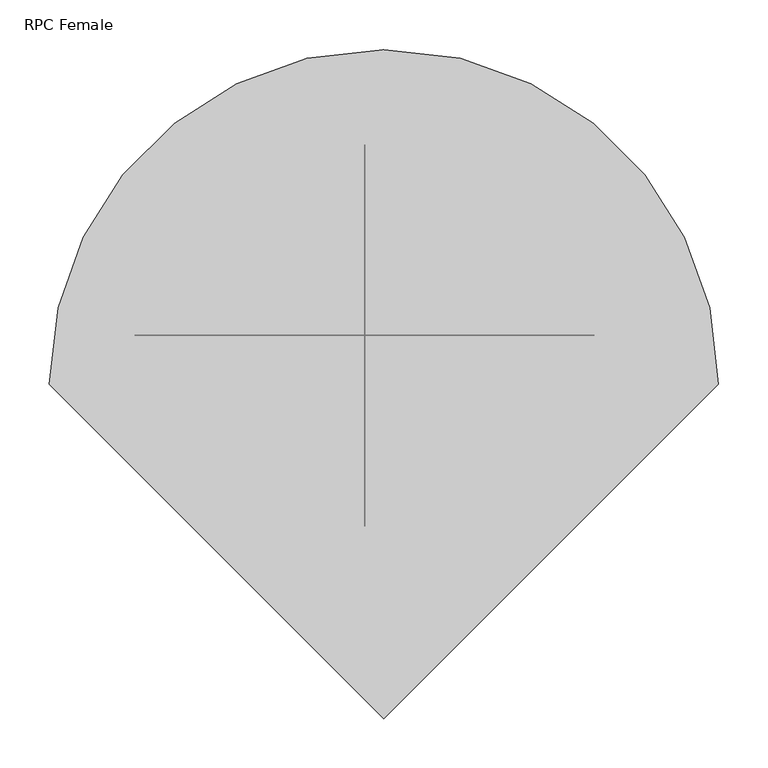
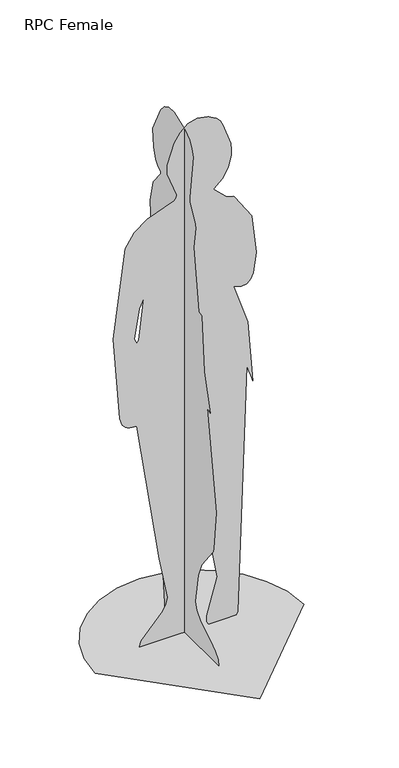
"""IFC4 building model written with IfcOpenShell, lengths in millimetres: proxy geometry, RPC Female : YinYin."""

import ifcopenshell
import ifcopenshell.guid

model = None  # the IFC model being written
_history = None  # IfcOwnerHistory: only IFC2X3 demands one
_inside = {}  # id of a spatial element -> (the spatial element, [elements in it])
_under = {}  # id of a project, library or spatial element -> (it, [spatial elements below it])
_declared = {}  # id of a project -> (the project, [libraries it declares])
_typed = {}  # id of a type object -> (the type object, [elements of that type])
_made_of = {}  # id of a material, layer set ... -> (it, [elements and type objects made of it])


def new_model(schema):
    """Start an empty IFC model of exactly this schema.

    Asked for "IFC4X3", IfcOpenShell would pick the latest addendum, in which some entities
    have other attributes; the version numbers below select the first issue.
    IFC2X3 requires an IfcOwnerHistory on every rooted entity: one is made here for all.
    """
    global model, _history
    if schema == "IFC4X3":
        model = ifcopenshell.file(schema_version=(4, 3, 0, 0))
    else:
        model = ifcopenshell.file(schema=schema)
    _inside.clear()
    _under.clear()
    _declared.clear()
    _typed.clear()
    _made_of.clear()
    _history = None
    if model.schema == "IFC2X3":
        org = make("IfcOrganization", Name="unknown")
        user = make(
            "IfcPersonAndOrganization",
            ThePerson=make("IfcPerson", FamilyName="unknown"),
            TheOrganization=org,
        )
        app = make(
            "IfcApplication",
            ApplicationDeveloper=org,
            Version="unknown",
            ApplicationFullName="unknown",
            ApplicationIdentifier="unknown",
        )
        _history = make(
            "IfcOwnerHistory",
            OwningUser=user,
            OwningApplication=app,
            ChangeAction="ADDED",
            CreationDate=0,
        )
    return model


def make(cls, **values):
    """One entity of the class cls with the attributes given. An attribute that is None is left unset."""
    return model.create_entity(
        cls, **{name: value for name, value in values.items() if value is not None}
    )


def rooted(cls, **values):
    """An entity with a GlobalId (a new one), such as an element, a storey or a relation."""
    return make(cls, GlobalId=ifcopenshell.guid.new(), OwnerHistory=_history, **values)


def si_unit(unit_type, name, prefix=None):
    """IfcSIUnit, for example si_unit("LENGTHUNIT", "METRE", prefix="MILLI")."""
    return make("IfcSIUnit", UnitType=unit_type, Prefix=prefix, Name=name)


def assignment(units):
    """IfcUnitAssignment: the units of a project."""
    return None if units is None else make("IfcUnitAssignment", Units=units)


def point(xyz):
    """IfcCartesianPoint."""
    return None if xyz is None else make("IfcCartesianPoint", Coordinates=xyz)


def direction(xyz):
    """IfcDirection."""
    return None if xyz is None else make("IfcDirection", DirectionRatios=xyz)


def frame(location, z_axis=None, x_axis=None):
    """IfcAxis2Placement3D, a coordinate frame: its origin and axes. An axis left out is left unset."""
    return make(
        "IfcAxis2Placement3D",
        Location=point(location),
        Axis=direction(z_axis),
        RefDirection=direction(x_axis),
    )


def origin():
    """The frame at (0, 0, 0) with its axes left unset."""
    return frame((0.0, 0.0, 0.0))


def place(relative_to, where):
    """IfcLocalPlacement: puts the frame where relative to a parent placement (None: the world)."""
    return make(
        "IfcLocalPlacement", PlacementRelTo=relative_to, RelativePlacement=where
    )


def context(
    kind, dimensions, precision=None, world=None, true_north=None, identifier=None
):
    """IfcGeometricRepresentationContext, for example the 3D "Model" context."""
    return make(
        "IfcGeometricRepresentationContext",
        ContextIdentifier=identifier,
        ContextType=kind,
        CoordinateSpaceDimension=dimensions,
        Precision=precision,
        WorldCoordinateSystem=world,
        TrueNorth=true_north,
    )


def project(units=None, contexts=None):
    """IfcProject with its units and contexts."""
    return rooted(
        "IfcProject",
        Name="project",
        RepresentationContexts=contexts,
        UnitsInContext=assignment(units),
    )


def spatial(cls, under=None, at=None, **own):
    """A site, building, storey or space (cls), placed at a placement, below another one or the project."""
    s = rooted(cls, ObjectPlacement=at, **own)
    if under is not None:
        _under.setdefault(under.id(), (under, []))[1].append(s)
    return s


def point_list(points):
    """IfcCartesianPointList2D or 3D."""
    cls = (
        "IfcCartesianPointList2D" if len(points[0]) == 2 else "IfcCartesianPointList3D"
    )
    return make(cls, CoordList=points)


def triangles(points, corners, closed=None, point_numbers=None):
    """IfcTriangulatedFaceSet: each triangle names its three corners, points numbered from 1."""
    return make(
        "IfcTriangulatedFaceSet",
        Coordinates=point_list(points),
        Closed=closed,
        CoordIndex=corners,
        PnIndex=point_numbers,
    )


def shape(context_of_items, identifier, shape_type, items):
    """IfcShapeRepresentation: the items that make up one representation, for example the "Body"."""
    return make(
        "IfcShapeRepresentation",
        ContextOfItems=context_of_items,
        RepresentationIdentifier=identifier,
        RepresentationType=shape_type,
        Items=items,
    )


def source(mapping_origin, context_of_items, identifier, shape_type, items):
    """IfcRepresentationMap: a shape defined once, which mapped items show again and again."""
    return make(
        "IfcRepresentationMap",
        MappingOrigin=mapping_origin,
        MappedRepresentation=shape(context_of_items, identifier, shape_type, items),
    )


def transform(
    local_origin,
    x_axis=None,
    y_axis=None,
    z_axis=None,
    scale=None,
    scale2=None,
    scale3=None,
    uniform=True,
):
    """IfcCartesianTransformationOperator3D, or its non-uniform kind. x_axis, y_axis, z_axis: its Axis1, 2, 3."""
    if uniform:
        return make(
            "IfcCartesianTransformationOperator3D",
            Axis1=direction(x_axis),
            Axis2=direction(y_axis),
            LocalOrigin=point(local_origin),
            Scale=scale,
            Axis3=direction(z_axis),
        )
    return make(
        "IfcCartesianTransformationOperator3DnonUniform",
        Axis1=direction(x_axis),
        Axis2=direction(y_axis),
        LocalOrigin=point(local_origin),
        Scale=scale,
        Axis3=direction(z_axis),
        Scale2=scale2,
        Scale3=scale3,
    )


def mapped(mapping_source, mapping_target):
    """IfcMappedItem: shows the shape of a source again, moved by a transform."""
    return make(
        "IfcMappedItem", MappingSource=mapping_source, MappingTarget=mapping_target
    )


def made_of(thing, what):
    """Note that an element or type object is made of a material, layer set ...; save() writes the relation."""
    if what is not None:
        _made_of.setdefault(what.id(), (what, []))[1].append(thing)
    return thing


def element(
    cls,
    number,
    at=None,
    inside=None,
    cuts=None,
    type_object=None,
    material=None,
    context=None,
    identifier="Body",
    shape_type=None,
    held_by="IfcProductDefinitionShape",
    body=None,
    shapes=None,
    **own,
):
    """One element of the class cls, such as IfcWall. Its Tag is "e" and its number.

    at: its placement. inside: the storey or other place that contains it. cuts: it is an
    opening in that element (IfcRelVoidsElement). A single representation is given by context,
    identifier, shape_type and body (its items); several are given by shapes. held_by: the class
    of the entity that holds the representations. save() writes the other relations.
    """
    e = rooted(cls, Tag="e%d" % number, ObjectPlacement=at, **own)
    if body is not None:
        shapes = [shape(context, identifier, shape_type, body)]
    if shapes is not None:
        e.Representation = make(held_by, Representations=shapes)
    if inside is not None:
        _inside.setdefault(inside.id(), (inside, []))[1].append(e)
    if cuts is not None:
        rooted(
            "IfcRelVoidsElement", RelatingBuildingElement=cuts, RelatedOpeningElement=e
        )
    if type_object is not None:
        _typed.setdefault(type_object.id(), (type_object, []))[1].append(e)
    return made_of(e, material)


def aggregate(whole, parts):
    """IfcRelAggregates: a whole, such as a stair, and the parts it consists of."""
    return rooted("IfcRelAggregates", RelatingObject=whole, RelatedObjects=parts)


def save(model, path):
    """Write the relations noted so far, then the file.

    IfcRelAggregates (storeys below a building ...), IfcRelContainedInSpatialStructure (elements
    in a storey), IfcRelDefinesByType, IfcRelAssociatesMaterial and IfcRelDeclares: one each for
    every whole, place, type object, material and project.
    """
    for whole, parts in _under.values():
        aggregate(whole, parts)
    for where, things in _inside.values():
        rooted(
            "IfcRelContainedInSpatialStructure",
            RelatedElements=things,
            RelatingStructure=where,
        )
    for kind, things in _typed.values():
        rooted("IfcRelDefinesByType", RelatedObjects=things, RelatingType=kind)
    for what, things in _made_of.values():
        rooted("IfcRelAssociatesMaterial", RelatedObjects=things, RelatingMaterial=what)
    for by, libraries in _declared.values():
        rooted("IfcRelDeclares", RelatingContext=by, RelatedDefinitions=libraries)
    model.write(path)


def rpc_female_6119fb87(model_context):
    return source(origin(), model_context, "Body", "Tessellation", [
        triangles([(-19.5611175, 62.5163331, 200.054177), (-19.5611152, 65.6149675, 206.6420561), (-19.5611152, 67.0930613, 208.6188795), (-19.561113, 68.5514434, 210.1580661), (-19.561113, 69.844742, 211.0626257), (-19.561113, 70.8275627, 211.135768), (-19.561113, 72.3678802, 205.9018034), (-19.561113, 74.2964098, 196.3806185), (-19.561113, 75.9138574, 184.6084991), (-19.561113, 76.5209197, 172.6210404), (-19.561113, 75.4182799, 162.4544372), (-19.561113, 71.9066574, 156.1446297), (-19.5611152, 65.2867172, 155.7276494), (-19.5611039, 157.7736182, 0.0), (-19.5611016, 193.0716999, 365.6725562), (-19.5611016, 178.8734568, 562.9772644), (-19.5610993, 217.6591707, 934.2117268), (-19.5610993, 211.3348838, 953.6969473), (-19.5610993, 209.2268184, 990.3578636), (-19.5610993, 217.6591707, 1061.6503143), (-19.5610993, 210.50601, 1080.5146425), (-19.5610993, 208.85929, 1098.4551172), (-19.5610971, 232.5501404, 1186.4916767), (-19.5610948, 242.5928596, 1369.1652649), (-19.5610993, 225.9704185, 1441.195752), (-19.5611016, 184.4143795, 1493.8335274), (-19.5611016, 184.4143795, 1502.144648), (-19.5610993, 199.7092126, 1513.6221451), (-19.5610993, 211.0346478, 1528.1208241), (-19.5610993, 224.1339935, 1563.6801361), (-19.5610993, 228.7409071, 1624.0425854), (-19.5611016, 183.9053081, 1715.3903526), (-19.5611039, 164.1472481, 1737.5990261), (-19.5611062, 139.3703811, 1750.94981), (-19.5611107, 108.0072428, 1752.6), (-19.5611175, 48.1994199, 1729.3935677), (-19.5611198, 20.4398407, 1708.5970173), (-19.5611198, 13.3301127, 1699.5173389), (-19.5611198, 7.887789, 1689.0607098), (-19.5611198, 0.7002218, 1662.8370197), (-19.5611198, 20.3545375, 1513.0532845), (-19.5611198, 18.6672041, 1499.3218552), (-19.5611198, -11.1306603, 1439.5698338), (-19.5611221, -14.5353557, 1426.8243908), (-19.5611198, -1.7222787, 1354.8805264), (-19.5611243, -31.6772816, 1150.3032606), (-19.5611266, -48.2997453, 1147.5328629), (-19.5611266, -62.8443699, 962.6950172), (-19.5611311, -95.3966934, 840.0179123), (-19.5611311, -94.2714078, 840.4783493), (-19.5611311, -92.0027327, 841.6656315), (-19.5611311, -89.0268515, 843.2890789), (-19.5611311, -85.779884, 845.057939), (-19.5611311, -82.69805, 846.6813864), (-19.5611311, -80.2174419, 847.8687412), (-19.5611311, -78.7742251, 848.3291056), (-19.5611357, -129.4408909, 519.2575856), (-19.5611334, -115.741718, 386.017608), (-19.5611334, -111.0109475, 373.0374773), (-19.5611266, -46.365175, 289.3376807), (-19.5611243, -27.5483094, 242.7219941), (-19.5611198, -11.1589414, 141.8756606), (-19.5611221, -19.6099427, 117.1299145), (-19.5611243, -40.4983047, 95.464113), (-19.5611289, -68.4628405, 75.9257889), (-19.5611311, -98.1422926, 57.5627155), (-19.5611357, -124.1755963, 39.4220441), (-19.5611357, -141.2014012, 20.5520522), (-19.5611357, -143.8586064, 0.0), (-183.0151008, 49.367172, 1064.4207121), (-167.6046679, 49.367172, 1163.5493271), (-152.5405437, 49.367172, 1194.6297701), (-168.2881109, 49.367172, 1056.0085802), (-175.1434882, 49.367172, 1046.9906713), (8.6640407, 49.3671675, 0.0), (3.1501566, 49.3671675, 32.2482746), (-2.0821968, 49.3671675, 69.3733591), (-6.8264337, 49.3671675, 108.190362), (-10.8760099, 49.3671675, 145.5140468), (-14.024312, 49.3671675, 178.1596922), (-16.0647898, 49.3671675, 202.9421185), (-16.7908537, 49.3671675, 216.6765999), (-12.1869764, 49.3671675, 219.1461257), (-0.3138061, 49.3671675, 225.0791757), (15.9209452, 49.3671675, 233.4869473), (33.6095424, 49.3671675, 243.3801843), (49.8442868, 49.3671629, 253.770157), (61.7174538, 49.3671629, 263.6679903), (66.3213379, 49.3671629, 272.0846822), (87.4456344, 49.3671629, 152.9572698), (53.4088494, 49.3671629, 31.0045278), (52.5814834, 49.3671629, 11.0292914), (59.1493465, 49.3671629, 0.0), (149.3171576, 49.3671584, 0.0), (152.8116755, 49.3671584, 10.4443548), (182.6784389, 49.3671584, 842.7883101), (184.325177, 49.3671584, 839.6736019), (187.3182356, 49.3671584, 831.6521439), (191.0744744, 49.3671584, 820.7077538), (195.0110255, 49.3671584, 808.8246128), (198.5446761, 49.3671584, 797.9861755), (201.0924312, 49.3671584, 790.1768412), (202.0712777, 49.3671584, 787.3802095), (185.4488367, 49.3671584, 995.1605501), (141.1223908, 49.3671584, 1130.9104036), (164.3033614, 49.3671584, 1124.3246864), (182.0565655, 49.3671584, 1128.1551939), (195.0604956, 49.3671584, 1140.1605658), (203.9936531, 49.3671584, 1158.0995871), (213.1529414, 49.3671584, 1225.1042908), (199.3009163, 49.3671584, 1355.3133488), (142.1371181, 49.3671584, 1439.8141502), (138.3520475, 49.3671584, 1443.9662224), (126.4536368, 49.3671629, 1446.4888882), (114.043366, 49.3671629, 1453.0155247), (76.6085234, 49.3671629, 1487.9363583), (74.6326765, 49.3671629, 1491.0630569), (103.0905098, 49.3671629, 1516.7510239), (122.0981614, 49.3671629, 1548.9569069), (131.6193734, 49.3671584, 1586.7359962), (132.8112338, 49.3671584, 1607.4201988), (130.0408452, 49.3671629, 1629.5832355), (105.4424193, 49.3671629, 1701.5050083), (96.1693025, 49.3671629, 1717.9445572), (84.0081807, 49.3671629, 1731.1446236), (55.2399058, 49.3671629, 1745.9405228), (21.127821, 49.3671675, 1752.5937504), (-8.6787592, 49.3671675, 1743.6800503), (-33.6906489, 49.3671675, 1722.8627163), (-53.4187143, 49.367172, 1693.8054783), (-75.0665981, 49.367172, 1625.6246109), (-76.0080877, 49.367172, 1593.8278599), (-45.7086335, 49.367172, 1512.9888988), (-45.9663349, 49.367172, 1502.7510063), (-52.5418193, 49.367172, 1494.1808899), (-141.4589345, 49.367172, 1463.3590794), (-183.2078579, 49.367172, 1431.0789276), (-212.1098365, 49.367172, 1385.7065517), (-252.2751901, 49.3671765, 1089.3543646), (-230.371785, 49.3671765, 807.1516771), (-222.5797643, 49.3671765, 783.138172), (-217.6561913, 49.3671765, 776.9216183), (-211.9299056, 49.367172, 771.9938667), (-205.4993388, 49.367172, 768.2337765), (-198.4630859, 49.367172, 765.520134), (-174.7038712, 49.367172, 762.4466297), (-101.5477987, 49.367172, 280.655816), (-74.3631844, 49.367172, 138.9321538), (-78.7405971, 49.367172, 117.6130336), (-91.1992752, 49.367172, 97.162465), (-159.9729389, 49.367172, 19.5097603), (-166.4325919, 49.367172, 0.0), (339.0977612, 6.67e-05, 0.0), (330.1330831, 77.6988366, 0.0), (304.601938, 149.0527116, 0.0), (264.5485507, 212.0173639, 0.0), (212.0174184, 264.5485688, 0.0), (149.0527207, 304.6018835, 0.0), (77.6988547, 330.1331194, 0.0), (0.0001125, 339.0977612, 0.000112), (-77.6986367, 330.1331194, 0.000112), (-149.0525208, 304.6018835, 0.000112), (-212.0171641, 264.5485507, 0.000112), (-264.5483871, 212.0174003, 0.0), (-304.6017018, 149.0526934, 0.0), (-330.132865, 77.6988093, 0.0), (-339.0975431, 7.37e-05, 0.0), (0.0001352, -339.0975795, 0.0)], [[14, 6, 7], [14, 7, 8], [14, 8, 9], [14, 9, 10], [14, 10, 11], [48, 49, 50], [48, 50, 51], [48, 51, 52], [48, 52, 53], [48, 53, 54], [48, 54, 55], [14, 11, 12], [69, 14, 12], [69, 12, 13], [68, 69, 13], [67, 68, 13], [66, 67, 13], [65, 66, 13], [64, 65, 13], [63, 64, 13], [62, 63, 13], [48, 55, 56], [62, 13, 1], [61, 62, 1], [46, 47, 48], [61, 1, 2], [61, 2, 3], [61, 3, 4], [61, 4, 5], [6, 14, 15], [5, 6, 15], [61, 5, 15], [60, 61, 15], [60, 15, 16], [59, 60, 16], [58, 59, 16], [57, 58, 16], [56, 57, 16], [48, 56, 16], [48, 16, 17], [48, 17, 18], [46, 48, 18], [46, 18, 19], [46, 19, 20], [46, 20, 21], [46, 21, 22], [46, 22, 23], [46, 23, 24], [45, 46, 24], [45, 24, 25], [45, 25, 26], [44, 45, 26], [43, 44, 26], [42, 43, 26], [41, 42, 26], [41, 26, 27], [41, 27, 28], [41, 28, 29], [41, 29, 30], [41, 30, 31], [40, 41, 31], [40, 31, 32], [39, 40, 32], [38, 39, 32], [37, 38, 32], [36, 37, 32], [35, 36, 32], [35, 32, 33], [34, 35, 33], [70, 75, 76], [70, 76, 77], [70, 77, 78], [70, 78, 79], [70, 79, 80], [70, 80, 81], [70, 81, 82], [74, 70, 82], [102, 103, 104], [101, 102, 104], [100, 101, 104], [99, 100, 104], [98, 99, 104], [97, 98, 104], [96, 97, 104], [151, 152, 75], [74, 82, 83], [74, 83, 84], [74, 84, 85], [74, 85, 86], [74, 86, 87], [74, 87, 88], [74, 88, 89], [150, 151, 75], [149, 150, 75], [93, 94, 95], [92, 93, 95], [91, 92, 95], [90, 91, 95], [90, 95, 96], [89, 90, 96], [74, 89, 96], [74, 96, 104], [73, 74, 104], [73, 104, 105], [72, 73, 105], [148, 149, 75], [148, 75, 70], [147, 148, 70], [146, 147, 70], [145, 146, 70], [144, 145, 70], [143, 144, 70], [142, 143, 70], [141, 142, 70], [140, 141, 70], [139, 140, 70], [139, 70, 71], [139, 71, 72], [138, 139, 72], [138, 72, 105], [137, 138, 105], [136, 137, 105], [135, 136, 105], [134, 135, 105], [134, 105, 106], [134, 106, 107], [134, 107, 108], [134, 108, 109], [134, 109, 110], [134, 110, 111], [134, 111, 112], [133, 134, 112], [112, 113, 114], [133, 112, 114], [133, 114, 115], [133, 115, 116], [133, 116, 117], [133, 117, 118], [133, 118, 119], [133, 119, 120], [133, 120, 121], [133, 121, 122], [132, 133, 122], [131, 132, 122], [130, 131, 122], [129, 130, 122], [129, 122, 123], [128, 129, 123], [127, 128, 123], [126, 127, 123], [126, 123, 124], [125, 126, 124], [167, 168, 153], [166, 167, 153], [166, 153, 154], [165, 166, 154], [165, 154, 155], [165, 155, 156], [164, 165, 156], [163, 164, 156], [163, 156, 157], [163, 157, 158], [163, 158, 159], [163, 159, 160], [163, 160, 161], [163, 161, 162]], closed=False),
    ])


if __name__ == "__main__":
    model = new_model("IFC4")
    model_context = context("Model", 3, world=origin())
    ifc_project = project(units=[si_unit("LENGTHUNIT", "METRE", prefix="MILLI")], contexts=[model_context])
    site = spatial("IfcSite", under=ifc_project)
    building = spatial("IfcBuilding", under=site)
    placement = place(None, origin())
    rpc_female_shape = rpc_female_6119fb87(model_context)
    element("IfcBuildingElementProxy", 1, Name="RPC Female : YinYin", ObjectType="RPC Female : YinYin", at=placement, inside=building, context=model_context, shape_type="MappedRepresentation", body=[
        mapped(rpc_female_shape, transform((0.0, 0.0, 0.0), x_axis=(1.0, 0.0, 0.0), y_axis=(0.0, 1.0, 0.0), z_axis=(0.0, 0.0, 1.0))),
    ])
    save(model, "model.ifc")

# Revit data of these elements
# Type "RPC Female : YinYin"
#   built-in parameter 1005198 = "{2, 15},{22, RPC-8-FUM5-CKXX-U6B5-E},{1, 0},{1, 0},{2, 15},{1, 8},{5, Color},{1, 0},{1, 0},{3, 0.8},{3, 0.8},{3, 0.8},{1, 8},{7, BBoxMin},{1, 0},{1, 0},{1, 0},{1, 0},{1, 0},{1, 8},{7, BBoxMax},{1, 0},{1, 0},{1, 0},{1, 0},{1, 0},{2, 11},{9, RPCTypeId},{1, 0},{1, 0},{22, RPC-8-FUM5-CKXX-U6B5-E},{1, 6},{14, RPCPlantHeight},{1, 0},{1, 0},{4, 5.75},{2, 11},{7, keyword},{1, 0},{1, 0},{35, :RPCs:People [Resorts]:Geometry:RPC},{2, 11},{8, category},{1, 0},{1, 0},{16, People [Resorts]},{2, 11},{12, LocalizedUID},{1, 0},{1, 0},{6, YinYin},{2, 14},{6, Height},{1, 0},{1, 0},{4, 5.75},{1, 2},{16, Cast Reflections},{1, 0},{1, 0},{1, 0},{1, 2},{6, Jitter},{1, 0},{1, 0},{1, 1},{1, 2},{9, Billboard},{1, 0},{1, 0},{1, 0},{1, 2},{12, Cast Shadows},{1, 0},{1, 0},{1, 1},{1, 2},{20, Apply Filter Effects},{1, 0},{1, 0},{1, 0},{2, 11},{28, Apply Filter Effects-Text-FC},{1, 0},{1, 0},{4, None},{21, assetlibrary_base.fbx},{1, 5},"
#   built-in parameter 1005195 = "RPC-8-FUM5-CKXX-U6B5-E"
#   Height = 0
